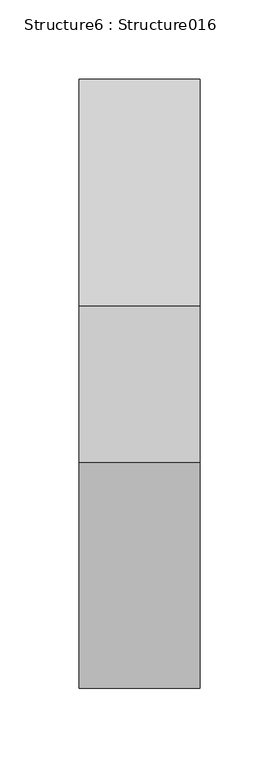
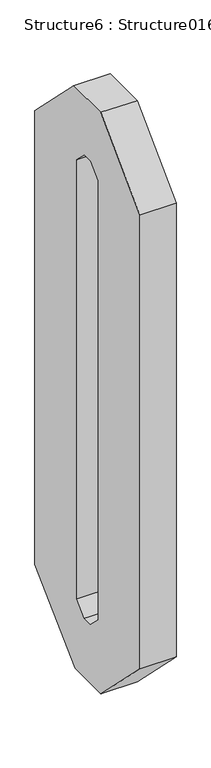
"""IFC4 building model written with IfcOpenShell, lengths in millimetres: proxy geometry, Structure6 : Structure016."""

from ifc_helpers import new_model, si_unit, frame, origin, place, context, project, spatial, polyline, outline, extrude, source, transform, mapped, element, save


def structure6_structure016_432a3f68(model_context):
    return source(origin(), model_context, "Body", "SweptSolid", [
        extrude(outline(polyline([(1013.3816076, 0.0), (1156.0607025, -142.6787371), (1156.0607025, -241.4608209), (1013.3819654, -384.139558), (-0.0016326, -384.1378636), (-142.5803241, -236.1624054), (-142.6787371, -142.6787371), (0.0, 0.0), (1013.3816076, 0.0)]), holes=[polyline([(-10.9769167, -203.0454249), (16.4629962, -230.4855986), (996.9085422, -230.4855986), (1024.3478687, -203.0462721), (1024.3478687, -181.0992162), (996.9085422, -153.6598897), (16.4632807, -153.6598897), (-10.9760695, -181.0992162), (-10.9769167, -203.0454249)])]), frame((-35624.0862846, 274854.897436, 4615.0263343), z_axis=(1.0, 0.0, 1.354250045437766e-12), x_axis=(-1.3542500454377577e-12, 0.0, 1.0)), (0.0, 0.0, 1.0), 76.2),
    ])


if __name__ == "__main__":
    model = new_model("IFC4")
    model_context = context("Model", 3, world=origin())
    ifc_project = project(units=[si_unit("LENGTHUNIT", "METRE", prefix="MILLI")], contexts=[model_context])
    site = spatial("IfcSite", under=ifc_project)
    building = spatial("IfcBuilding", under=site)
    placement = place(None, origin())
    structure6_structure016_shape = structure6_structure016_432a3f68(model_context)
    element("IfcBuildingElementProxy", 1, Name="Structure6 : Structure016", ObjectType="Structure6 : Structure016", at=placement, inside=building, context=model_context, shape_type="MappedRepresentation", body=[
        mapped(structure6_structure016_shape, transform((0.0, 0.0, 0.0), x_axis=(1.0, 0.0, 0.0), y_axis=(0.0, 1.0, 0.0), z_axis=(0.0, 0.0, 1.0))),
    ])
    save(model, "model.ifc")

# Revit data of these elements
# Type "Structure6 : Structure016"
#   NameOverride = "Structure016"
# Element 1 (IfcBuildingElementProxy, "Structure6 : Structure016")
#   Materials on its faces: "BRUSHED ALUMINUM LETTERING"
# Materials
#   "BRUSHED ALUMINUM LETTERING": class "Unassigned", colour RGB 169 181 186, transparency 0, Cost = 0
